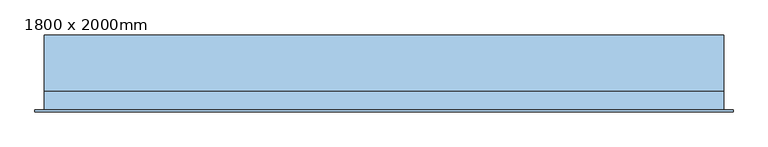
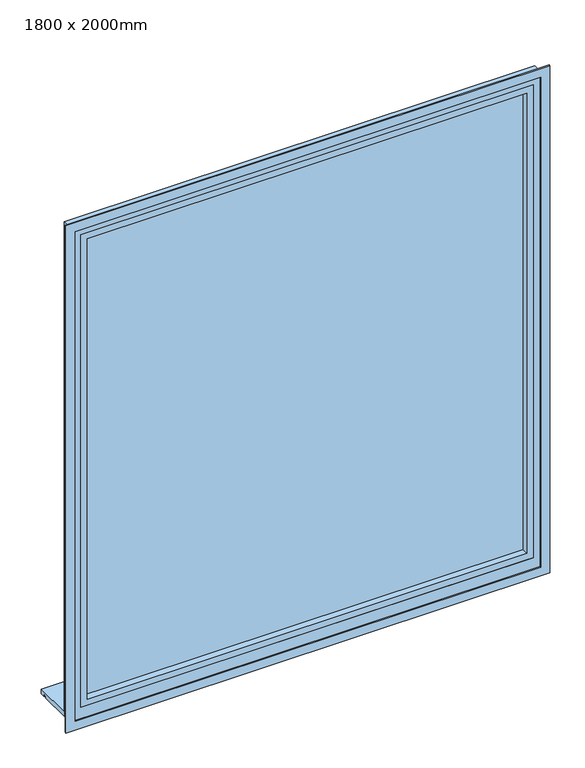
"""IFC4 building model written with IfcOpenShell, lengths in millimetres: window geometry, Ventana simple fija con cubrejuntas interior : 1800 x 2000mm."""

from ifc_helpers import new_model, si_unit, frame, origin, place, context, project, spatial, polyline, outline, extrude, faceted_brep, source, transform, mapped, element, save


def window_1800_x_2000mm_da90d486(model_context):
    return source(origin(), model_context, "Body", "SolidModel", [
        extrude(outline(polyline([(125.0, 920.0), (125.0, 900.0), (105.0, 900.0), (105.0, 910.0), (95.0, 910.0), (95.0, 900.0), (-25.0, 900.0), (-25.0, 920.0), (125.0, 920.0)])), frame((-900.0, 0.0, 0.0), z_axis=(1.0, 0.0, 0.0), x_axis=(0.0, 1.0, 0.0)), (0.0, 0.0, 1.0), 1800.0),
        extrude(outline(polyline([(-855.0, -49.0), (-855.0, -35.0), (855.0, -35.0), (855.0, -49.0), (-855.0, -49.0)])), frame((0.0, 0.0, 965.0), z_axis=(0.0, 0.0, 1.0), x_axis=(1.0, 0.0, 0.0)), (0.0, 0.0, 1.0), 1890.0),
        extrude(outline(polyline([(2865.0, -865.0), (955.0, -865.0), (955.0, 865.0), (2865.0, 865.0), (2865.0, -865.0)]), holes=[polyline([(2840.0, 840.0), (980.0, 840.0), (980.0, -840.0), (2840.0, -840.0), (2840.0, 840.0)])]), frame((0.0, -75.0, 0.0), z_axis=(0.0, 1.0, 0.0), x_axis=(0.0, 0.0, 1.0)), (0.0, 0.0, 1.0), 26.0),
        faceted_brep([(900.0, -25.0, 2900.0), (900.0, -75.0, 2900.0), (900.0, -75.0, 900.0), (900.0, -25.0, 900.0), (-900.0, -75.0, 2900.0), (-900.0, -75.0, 900.0), (-865.0, -75.0, 2865.0), (865.0, -75.0, 2865.0), (865.0, -75.0, 955.0), (-865.0, -75.0, 955.0), (-900.0, -25.0, 900.0), (-900.0, -25.0, 2900.0), (840.0, -25.0, 2840.0), (-840.0, -25.0, 2840.0), (-840.0, -25.0, 980.0), (840.0, -25.0, 980.0), (840.0, -35.0, 2840.0), (840.0, -35.0, 980.0), (-840.0, -35.0, 980.0), (865.0, -35.0, 2865.0), (-865.0, -35.0, 2865.0), (-865.0, -35.0, 955.0), (865.0, -35.0, 955.0), (-840.0, -35.0, 2840.0)], [[[0, 1, 2, 3]], [[2, 1, 4, 5], [6, 7, 8, 9]], [[5, 10, 3, 2]], [[10, 11, 0, 3], [12, 13, 14, 15]], [[16, 12, 15, 17]], [[17, 15, 14, 18]], [[19, 20, 21, 22], [23, 16, 17, 18]], [[7, 19, 22, 8]], [[8, 22, 21, 9]], [[13, 23, 18, 14]], [[20, 6, 9, 21]], [[4, 11, 10, 5]], [[11, 4, 1, 0]], [[23, 13, 12, 16]], [[6, 20, 19, 7]]]),
        extrude(outline(polyline([(2925.0, -925.0), (875.0, -925.0), (875.0, 925.0), (2925.0, 925.0), (2925.0, -925.0)]), holes=[polyline([(2890.0, 890.0), (910.0, 890.0), (910.0, -890.0), (2890.0, -890.0), (2890.0, 890.0)])]), frame((0.0, -80.0, 0.0), z_axis=(0.0, 1.0, 0.0), x_axis=(0.0, 0.0, 1.0)), (0.0, 0.0, 1.0), 5.0),
    ])


if __name__ == "__main__":
    model = new_model("IFC4")
    model_context = context("Model", 3, world=origin())
    ifc_project = project(units=[si_unit("LENGTHUNIT", "METRE", prefix="MILLI")], contexts=[model_context])
    site = spatial("IfcSite", under=ifc_project)
    building = spatial("IfcBuilding", under=site)
    placement = place(None, origin())
    window_1800_x_2000mm_shape = window_1800_x_2000mm_da90d486(model_context)
    element("IfcWindow", 1, ObjectType="Ventana simple fija con cubrejuntas interior : 1800 x 2000mm", at=placement, inside=building, context=model_context, shape_type="MappedRepresentation", body=[
        mapped(window_1800_x_2000mm_shape, transform((0.0, 0.0, 0.0), x_axis=(1.0, 0.0, 0.0), y_axis=(0.0, 1.0, 0.0), z_axis=(0.0, 0.0, 1.0))),
    ])
    save(model, "model.ifc")

# Revit data of these elements
# Type "Ventana simple fija con cubrejuntas interior : 1800 x 2000mm"
#   Type Mark = "42"
#   Construction Type Id = "GSP4R"
#   Analytic Construction = "1/8 en cristalera simple Pilkington"
#   Grosor de pared [instance default] = 0.20 m
#   W1 = 1.68 m
#   Visual Light Transmittance = 0.9
#   Anchura de cubrejuntas = 0.035 m
#   Grosor de cubrejuntas = 0.005 m
#   Solar Heat Gain Coefficient = 0.78
#   Grosor de antepecho = 0.02 m
#   Profundidad de antepecho [instance default] = 0.20 m
#   Rough Width = 1.80 m
#   Rough Height = 2.00 m
#   Height = 2.00 m
#   Heat Transfer Coefficient (U) = 3.6886 W/(m²·K)
#   Anchura de marco = 0.06 m
#   Grosor de marco = 0.05 m
#   Anchura de batiente de alzado = 0.50 m
#   Distancia entre antepecho y muro = 0.05 m
#   Altura de antepecho por defecto = 0.90 m
#   Width = 1.80 m
#   Define Thermal Properties by = 1
#   Material de antepecho = none
#   Material de cristalera = Vidrio
#   Material de estructura = none
#   Wall Closure = (empty or 0)
# Element 1 (IfcWindow, "Ventana simple fija con cubrejuntas interior : 1800 x 2000mm")
#   Grosor de pared = 0.15 m
#   Profundidad de antepecho = 0.15 m
#   Materials on its faces: "Vidrio"
# Materials
#   "Vidrio": class "Vidrio", colour RGB 245 245 243, transparency 1, Description = "Vidrio de cal sodada", Cost = 0
